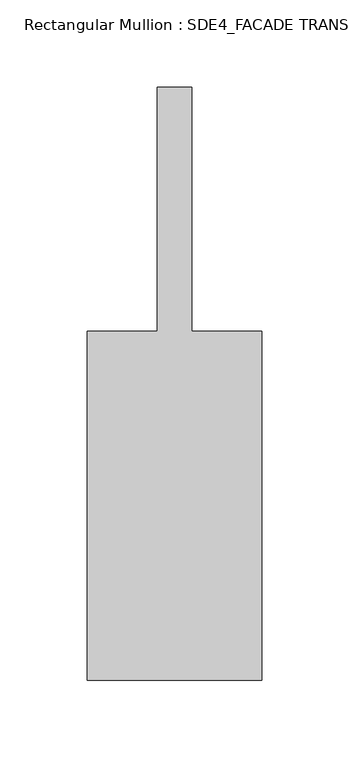
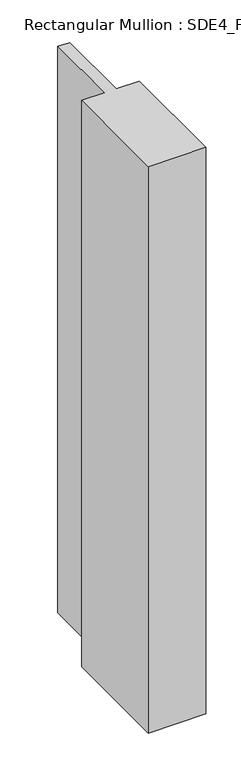
"""IFC4 building model written with IfcOpenShell, lengths in millimetres: member geometry, Rectangular Mullion : SDE4_FACADE TRANSOM TYPE 1."""

import ifcopenshell
import ifcopenshell.guid

model = None  # the IFC model being written
_history = None  # IfcOwnerHistory: only IFC2X3 demands one
_inside = {}  # id of a spatial element -> (the spatial element, [elements in it])
_under = {}  # id of a project, library or spatial element -> (it, [spatial elements below it])
_declared = {}  # id of a project -> (the project, [libraries it declares])
_typed = {}  # id of a type object -> (the type object, [elements of that type])
_made_of = {}  # id of a material, layer set ... -> (it, [elements and type objects made of it])


def new_model(schema):
    """Start an empty IFC model of exactly this schema.

    Asked for "IFC4X3", IfcOpenShell would pick the latest addendum, in which some entities
    have other attributes; the version numbers below select the first issue.
    IFC2X3 requires an IfcOwnerHistory on every rooted entity: one is made here for all.
    """
    global model, _history
    if schema == "IFC4X3":
        model = ifcopenshell.file(schema_version=(4, 3, 0, 0))
    else:
        model = ifcopenshell.file(schema=schema)
    _inside.clear()
    _under.clear()
    _declared.clear()
    _typed.clear()
    _made_of.clear()
    _history = None
    if model.schema == "IFC2X3":
        org = make("IfcOrganization", Name="unknown")
        user = make(
            "IfcPersonAndOrganization",
            ThePerson=make("IfcPerson", FamilyName="unknown"),
            TheOrganization=org,
        )
        app = make(
            "IfcApplication",
            ApplicationDeveloper=org,
            Version="unknown",
            ApplicationFullName="unknown",
            ApplicationIdentifier="unknown",
        )
        _history = make(
            "IfcOwnerHistory",
            OwningUser=user,
            OwningApplication=app,
            ChangeAction="ADDED",
            CreationDate=0,
        )
    return model


def make(cls, **values):
    """One entity of the class cls with the attributes given. An attribute that is None is left unset."""
    return model.create_entity(
        cls, **{name: value for name, value in values.items() if value is not None}
    )


def rooted(cls, **values):
    """An entity with a GlobalId (a new one), such as an element, a storey or a relation."""
    return make(cls, GlobalId=ifcopenshell.guid.new(), OwnerHistory=_history, **values)


def si_unit(unit_type, name, prefix=None):
    """IfcSIUnit, for example si_unit("LENGTHUNIT", "METRE", prefix="MILLI")."""
    return make("IfcSIUnit", UnitType=unit_type, Prefix=prefix, Name=name)


def assignment(units):
    """IfcUnitAssignment: the units of a project."""
    return None if units is None else make("IfcUnitAssignment", Units=units)


def point(xyz):
    """IfcCartesianPoint."""
    return None if xyz is None else make("IfcCartesianPoint", Coordinates=xyz)


def direction(xyz):
    """IfcDirection."""
    return None if xyz is None else make("IfcDirection", DirectionRatios=xyz)


def frame(location, z_axis=None, x_axis=None):
    """IfcAxis2Placement3D, a coordinate frame: its origin and axes. An axis left out is left unset."""
    return make(
        "IfcAxis2Placement3D",
        Location=point(location),
        Axis=direction(z_axis),
        RefDirection=direction(x_axis),
    )


def origin():
    """The frame at (0, 0, 0) with its axes left unset."""
    return frame((0.0, 0.0, 0.0))


def place(relative_to, where):
    """IfcLocalPlacement: puts the frame where relative to a parent placement (None: the world)."""
    return make(
        "IfcLocalPlacement", PlacementRelTo=relative_to, RelativePlacement=where
    )


def context(
    kind, dimensions, precision=None, world=None, true_north=None, identifier=None
):
    """IfcGeometricRepresentationContext, for example the 3D "Model" context."""
    return make(
        "IfcGeometricRepresentationContext",
        ContextIdentifier=identifier,
        ContextType=kind,
        CoordinateSpaceDimension=dimensions,
        Precision=precision,
        WorldCoordinateSystem=world,
        TrueNorth=true_north,
    )


def project(units=None, contexts=None):
    """IfcProject with its units and contexts."""
    return rooted(
        "IfcProject",
        Name="project",
        RepresentationContexts=contexts,
        UnitsInContext=assignment(units),
    )


def spatial(cls, under=None, at=None, **own):
    """A site, building, storey or space (cls), placed at a placement, below another one or the project."""
    s = rooted(cls, ObjectPlacement=at, **own)
    if under is not None:
        _under.setdefault(under.id(), (under, []))[1].append(s)
    return s


def polyline(points):
    """IfcPolyline through the points."""
    return make("IfcPolyline", Points=[point(p) for p in points])


def outline(outer, holes=None, kind="AREA"):
    """IfcArbitraryClosedProfileDef: a profile drawn as a closed curve; with holes, ...WithVoids."""
    if holes is None:
        return make("IfcArbitraryClosedProfileDef", ProfileType=kind, OuterCurve=outer)
    return make(
        "IfcArbitraryProfileDefWithVoids",
        ProfileType=kind,
        OuterCurve=outer,
        InnerCurves=holes,
    )


def extrude(swept, where, along, depth):
    """IfcExtrudedAreaSolid: the profile swept, set in the frame where, extruded along a direction by depth."""
    return make(
        "IfcExtrudedAreaSolid",
        SweptArea=swept,
        Position=where,
        ExtrudedDirection=direction(along),
        Depth=depth,
    )


def shape(context_of_items, identifier, shape_type, items):
    """IfcShapeRepresentation: the items that make up one representation, for example the "Body"."""
    return make(
        "IfcShapeRepresentation",
        ContextOfItems=context_of_items,
        RepresentationIdentifier=identifier,
        RepresentationType=shape_type,
        Items=items,
    )


def source(mapping_origin, context_of_items, identifier, shape_type, items):
    """IfcRepresentationMap: a shape defined once, which mapped items show again and again."""
    return make(
        "IfcRepresentationMap",
        MappingOrigin=mapping_origin,
        MappedRepresentation=shape(context_of_items, identifier, shape_type, items),
    )


def transform(
    local_origin,
    x_axis=None,
    y_axis=None,
    z_axis=None,
    scale=None,
    scale2=None,
    scale3=None,
    uniform=True,
):
    """IfcCartesianTransformationOperator3D, or its non-uniform kind. x_axis, y_axis, z_axis: its Axis1, 2, 3."""
    if uniform:
        return make(
            "IfcCartesianTransformationOperator3D",
            Axis1=direction(x_axis),
            Axis2=direction(y_axis),
            LocalOrigin=point(local_origin),
            Scale=scale,
            Axis3=direction(z_axis),
        )
    return make(
        "IfcCartesianTransformationOperator3DnonUniform",
        Axis1=direction(x_axis),
        Axis2=direction(y_axis),
        LocalOrigin=point(local_origin),
        Scale=scale,
        Axis3=direction(z_axis),
        Scale2=scale2,
        Scale3=scale3,
    )


def mapped(mapping_source, mapping_target):
    """IfcMappedItem: shows the shape of a source again, moved by a transform."""
    return make(
        "IfcMappedItem", MappingSource=mapping_source, MappingTarget=mapping_target
    )


def made_of(thing, what):
    """Note that an element or type object is made of a material, layer set ...; save() writes the relation."""
    if what is not None:
        _made_of.setdefault(what.id(), (what, []))[1].append(thing)
    return thing


def element(
    cls,
    number,
    at=None,
    inside=None,
    cuts=None,
    type_object=None,
    material=None,
    context=None,
    identifier="Body",
    shape_type=None,
    held_by="IfcProductDefinitionShape",
    body=None,
    shapes=None,
    **own,
):
    """One element of the class cls, such as IfcWall. Its Tag is "e" and its number.

    at: its placement. inside: the storey or other place that contains it. cuts: it is an
    opening in that element (IfcRelVoidsElement). A single representation is given by context,
    identifier, shape_type and body (its items); several are given by shapes. held_by: the class
    of the entity that holds the representations. save() writes the other relations.
    """
    e = rooted(cls, Tag="e%d" % number, ObjectPlacement=at, **own)
    if body is not None:
        shapes = [shape(context, identifier, shape_type, body)]
    if shapes is not None:
        e.Representation = make(held_by, Representations=shapes)
    if inside is not None:
        _inside.setdefault(inside.id(), (inside, []))[1].append(e)
    if cuts is not None:
        rooted(
            "IfcRelVoidsElement", RelatingBuildingElement=cuts, RelatedOpeningElement=e
        )
    if type_object is not None:
        _typed.setdefault(type_object.id(), (type_object, []))[1].append(e)
    return made_of(e, material)


def aggregate(whole, parts):
    """IfcRelAggregates: a whole, such as a stair, and the parts it consists of."""
    return rooted("IfcRelAggregates", RelatingObject=whole, RelatedObjects=parts)


def save(model, path):
    """Write the relations noted so far, then the file.

    IfcRelAggregates (storeys below a building ...), IfcRelContainedInSpatialStructure (elements
    in a storey), IfcRelDefinesByType, IfcRelAssociatesMaterial and IfcRelDeclares: one each for
    every whole, place, type object, material and project.
    """
    for whole, parts in _under.values():
        aggregate(whole, parts)
    for where, things in _inside.values():
        rooted(
            "IfcRelContainedInSpatialStructure",
            RelatedElements=things,
            RelatingStructure=where,
        )
    for kind, things in _typed.values():
        rooted("IfcRelDefinesByType", RelatedObjects=things, RelatingType=kind)
    for what, things in _made_of.values():
        rooted("IfcRelAssociatesMaterial", RelatedObjects=things, RelatingMaterial=what)
    for by, libraries in _declared.values():
        rooted("IfcRelDeclares", RelatingContext=by, RelatedDefinitions=libraries)
    model.write(path)


def rectangular_mullion_sde4_facade_transom_type_1_5b9f8211(model_context):
    return source(origin(), model_context, "Body", "SweptSolid", [
        extrude(outline(polyline([(50.0, -132.5), (-50.0, -132.5), (-50.0, 67.5), (-10.0, 67.5), (-10.0, 207.5), (10.0, 207.5), (10.0, 67.5), (50.0, 67.5), (50.0, -132.5)])), frame((0.0, 0.0, -1038.0), z_axis=(0.0, 0.0, 1.0), x_axis=(1.0, 0.0, 0.0)), (0.0, 0.0, 1.0), 1038.0),
    ])


if __name__ == "__main__":
    model = new_model("IFC4")
    model_context = context("Model", 3, world=origin())
    ifc_project = project(units=[si_unit("LENGTHUNIT", "METRE", prefix="MILLI")], contexts=[model_context])
    site = spatial("IfcSite", under=ifc_project)
    building = spatial("IfcBuilding", under=site)
    placement = place(None, origin())
    rectangular_mullion_sde4_facade_transom_type_1_shape = rectangular_mullion_sde4_facade_transom_type_1_5b9f8211(model_context)
    element("IfcMember", 1, ObjectType="Rectangular Mullion : SDE4_FACADE TRANSOM TYPE 1", at=placement, inside=building, context=model_context, shape_type="MappedRepresentation", body=[
        mapped(rectangular_mullion_sde4_facade_transom_type_1_shape, transform((0.0, 0.0, 0.0), x_axis=(1.0, 0.0, 0.0), y_axis=(0.0, 1.0, 0.0), z_axis=(0.0, 0.0, 1.0))),
    ])
    save(model, "model.ifc")

# Revit data of these elements
# Type "Rectangular Mullion : SDE4_FACADE TRANSOM TYPE 1"
#   built-in parameter 1007322 = 1.11549 (stored number, unit not read)
#   built-in parameter 1007321 = 0.164042 (stored number, unit not read)
#   built-in parameter 1007320 = 0.164042 (stored number, unit not read)
